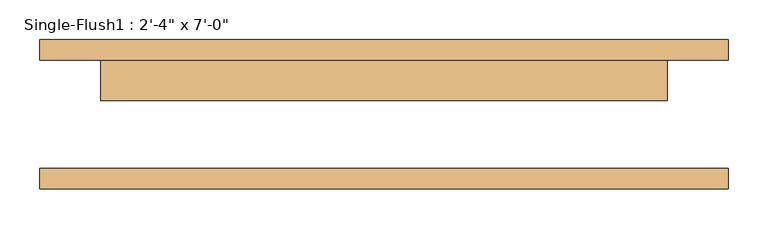
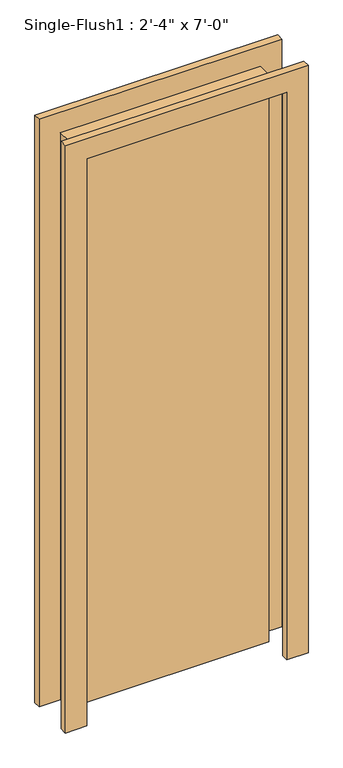
"""IFC4 building model written with IfcOpenShell, lengths in millimetres: door geometry."""

from ifc_helpers import new_model, si_unit, frame, origin, origin_with_axes, place, context, project, spatial, polyline, outline, extrude, source, transform, mapped, element, save


def door_eeaf238e(model_context):
    return source(origin(), model_context, "Body", "SweptSolid", [
        extrude(outline(polyline([(2209.8, -431.8), (0.0, -431.8), (0.0, -355.6), (2133.6, -355.6), (2133.6, 355.6), (0.0, 355.6), (0.0, 431.8), (2209.8, 431.8), (2209.8, -431.8)])), frame((0.0, 68.2625, 0.0), z_axis=(0.0, 1.0, 0.0), x_axis=(0.0, 0.0, 1.0)), (0.0, 0.0, 1.0), 25.4),
        extrude(outline(polyline([(2209.8, 431.8), (2209.8, -431.8), (0.0, -431.8), (0.0, -355.6), (2133.6, -355.6), (2133.6, 355.6), (0.0, 355.6), (0.0, 431.8), (2209.8, 431.8)])), frame((0.0, -93.6625, 0.0), z_axis=(0.0, 1.0, 0.0), x_axis=(0.0, 0.0, 1.0)), (0.0, 0.0, 1.0), 25.4),
        extrude(outline(polyline([(355.6, 17.4625), (-355.6, 17.4625), (-355.6, 68.2625), (355.6, 68.2625), (355.6, 17.4625)])), origin_with_axes(), (0.0, 0.0, 1.0), 2133.6),
    ])


if __name__ == "__main__":
    model = new_model("IFC4")
    model_context = context("Model", 3, world=origin())
    ifc_project = project(units=[si_unit("LENGTHUNIT", "METRE", prefix="MILLI")], contexts=[model_context])
    site = spatial("IfcSite", under=ifc_project)
    building = spatial("IfcBuilding", under=site)
    placement = place(None, origin())
    door_shape = door_eeaf238e(model_context)
    element("IfcDoor", 1, ObjectType="Single-Flush1 : 2'-4\" x 7'-0\"", at=placement, inside=building, context=model_context, shape_type="MappedRepresentation", body=[
        mapped(door_shape, transform((0.0, 0.0, 0.0), x_axis=(1.0, 0.0, 0.0), y_axis=(0.0, 1.0, 0.0), z_axis=(0.0, 0.0, 1.0))),
    ])
    save(model, "model.ifc")

# Revit data of these elements
# Type "Single-Flush1 : 2'-4\" x 7'-0\""
#   Type Mark = "D2"
#   Construction Type Id = "MDOOR"
#   Assembly Code = "C1020"
#   Analytic Construction = "Metal"
#   Thickness = 0' - 2"
#   Heat Transfer Coefficient (U) = 3.7021 W/(m²·K)
#   Height = 7' - 0"
#   Trim Projection Ext = 0' - 1"
#   Trim Projection Int = 0' - 1"
#   Trim Width = 0' - 3"
#   Width = 2' - 4"
#   Door Material = Door - Panel
#   Frame Material = Door - Frame
#   Visual Light Transmittance = 0
#   Solar Heat Gain Coefficient = 0
#   Function = (empty or 0)
#   Wall Closure = (empty or 0)
# Element 1 (IfcDoor, "Single-Flush1 : 2'-4\" x 7'-0\"")
#   Materials on its faces: "Door - Frame", "Door - Panel"
# Materials
#   "Door - Panel": class "Wood", colour RGB 210 159 95, transparency 0, Cost = 0
#   "Door - Frame": class "Miscellaneous", colour RGB 118 70 51, transparency 0, Cost = 0
